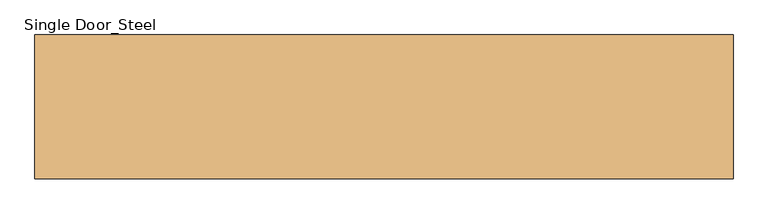
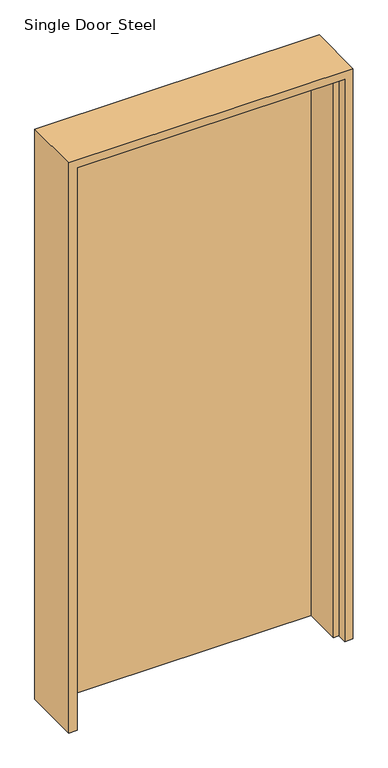
"""IFC4 building model written with IfcOpenShell, lengths in millimetres: door geometry, Single Door_Steel : H_DR_AR B12_Door_Single FSD 01."""

from ifc_helpers import new_model, si_unit, origin, origin_with_axes, place, context, project, spatial, polyline, outline, extrude, faceted_brep, source, transform, mapped, element, save


def single_door_steel_ed84bdaa(model_context):
    return source(origin(), model_context, "Body", "SolidModel", [
        extrude(outline(polyline([(480.0, 105.0), (480.0, 70.0), (-480.0, 70.0), (-480.0, 105.0), (480.0, 105.0)])), origin_with_axes(), (0.0, 0.0, 1.0), 2130.0),
        faceted_brep([(480.0, 105.0, 0.0), (510.0, 105.0, 0.0), (510.0, -105.0, 0.0), (480.0, -105.0, 0.0), (480.0, -70.0, 0.0), (460.0, -70.0, 0.0), (460.0, 70.0, 0.0), (480.0, 70.0, 0.0), (480.0, 105.0, 2130.0), (-480.0, 105.0, 2130.0), (-480.0, 105.0, 0.0), (-510.0, 105.0, 0.0), (-510.0, 105.0, 2160.0), (510.0, 105.0, 2160.0), (510.0, -105.0, 2160.0), (-510.0, -105.0, 2160.0), (-510.0, -105.0, 0.0), (-480.0, -105.0, 0.0), (-480.0, -105.0, 2130.0), (480.0, -105.0, 2130.0), (480.0, -70.0, 2130.0), (-480.0, -70.0, 2130.0), (-480.0, -70.0, 0.0), (-460.0, -70.0, 0.0), (-460.0, -70.0, 2110.0), (460.0, -70.0, 2110.0), (460.0, 70.0, 2110.0), (-460.0, 70.0, 2110.0), (-460.0, 70.0, 0.0), (-480.0, 70.0, 0.0), (-480.0, 70.0, 2130.0), (480.0, 70.0, 2130.0)], [[[0, 1, 2, 3, 4, 5, 6, 7]], [[1, 0, 8, 9, 10, 11, 12, 13]], [[2, 1, 13, 14]], [[3, 2, 14, 15, 16, 17, 18, 19]], [[4, 3, 19, 20]], [[5, 4, 20, 21, 22, 23, 24, 25]], [[6, 5, 25, 26]], [[7, 6, 26, 27, 28, 29, 30, 31]], [[0, 7, 31, 8]], [[9, 30, 29, 10]], [[10, 29, 28, 23, 22, 17, 16, 11]], [[15, 12, 11, 16]], [[21, 18, 17, 22]], [[27, 24, 23, 28]], [[14, 13, 12, 15]], [[20, 19, 18, 21]], [[26, 25, 24, 27]], [[8, 31, 30, 9]]]),
    ])


if __name__ == "__main__":
    model = new_model("IFC4")
    model_context = context("Model", 3, world=origin())
    ifc_project = project(units=[si_unit("LENGTHUNIT", "METRE", prefix="MILLI")], contexts=[model_context])
    site = spatial("IfcSite", under=ifc_project)
    building = spatial("IfcBuilding", under=site)
    placement = place(None, origin())
    single_door_steel_shape = single_door_steel_ed84bdaa(model_context)
    element("IfcDoor", 1, ObjectType="Single Door_Steel : H_DR_AR B12_Door_Single FSD 01", at=placement, inside=building, context=model_context, shape_type="MappedRepresentation", body=[
        mapped(single_door_steel_shape, transform((0.0, 0.0, 0.0), x_axis=(1.0, 0.0, 0.0), y_axis=(0.0, 1.0, 0.0), z_axis=(0.0, 0.0, 1.0))),
    ])
    save(model, "model.ifc")

# Revit data of these elements
# Type "Single Door_Steel : H_DR_AR B12_Door_Single FSD 01"
#   Type Mark = "FRD"
#   Analytic Construction = "<None>"
#   프레임 투영 외부. = 25 mm
#   프레임 투영 내부. = 25 mm
#   프레임 폭 = 75 mm
#   Height = 2160 mm
#   Width = 1020 mm
#   Define Thermal Properties by = 1
#   문 패널 = none
#   문 프레임 = none
#   Function = (empty or 0)
#   Wall Closure = (empty or 0)
